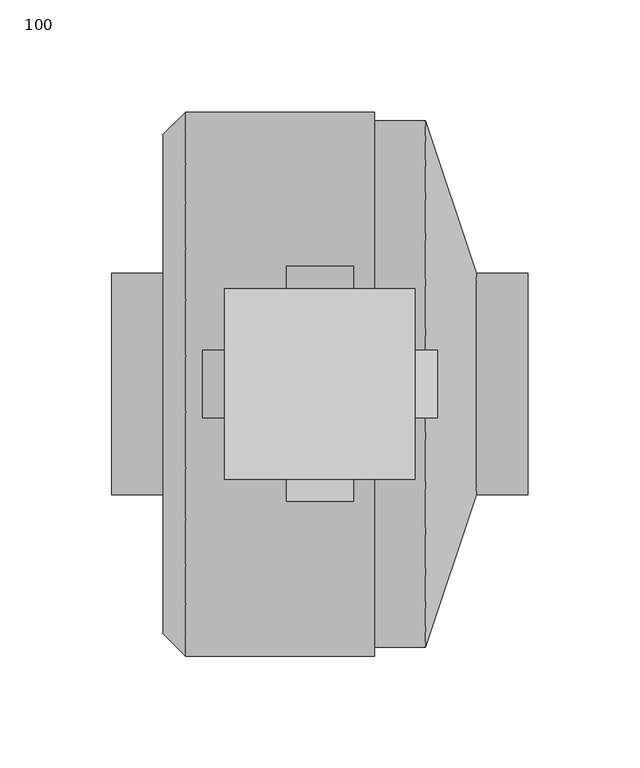
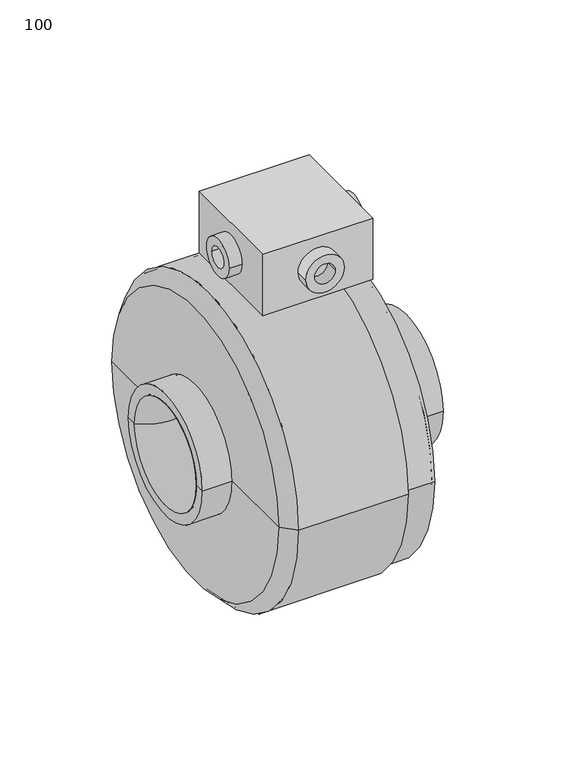
"""IFC4 building model written with IfcOpenShell, lengths in millimetres: proxy geometry, ВЕЗА_Канал-ВЕНТ : 100."""

from ifc_helpers import new_model, si_unit, point, frame, frame_2d, origin, place, context, project, spatial, polyline, circle_curve, ellipse_curve, trimmed, segment, composite_curve, outline, extrude, source, transform, mapped, element, save
from ifc_brep_helpers import plane_surface, cylinder_surface, revolved_surface, advanced_brep


def proxy_100_a4e0c5e0(model_context):
    return source(origin(), model_context, "Body", "SolidModel", [
        extrude(outline(composite_curve([segment(trimmed(circle_curve(frame_2d((0.0, 147.0)), 15.0), [point((-15.0, 147.0))], [point((15.0, 147.0))], False, "CARTESIAN"), True, "CONTINUOUS"), segment(trimmed(circle_curve(frame_2d((0.0, 147.0)), 15.0), [point((15.0, 147.0))], [point((-15.0, 147.0))], False, "CARTESIAN"), True, "CONTINUOUS")], self_intersect=False), holes=[composite_curve([segment(trimmed(circle_curve(frame_2d((0.0, 147.0)), 8.0), [point((-8.0, 147.0))], [point((8.0, 147.0))], True, "CARTESIAN"), True, "CONTINUOUS"), segment(trimmed(circle_curve(frame_2d((0.0, 147.0)), 8.0), [point((8.0, 147.0))], [point((-8.0, 147.0))], True, "CARTESIAN"), True, "CONTINUOUS")], self_intersect=False)]), frame((42.5, 0.0, 0.0), z_axis=(1.0, 0.0, 0.0), x_axis=(0.0, 1.0, 0.0)), (0.0, 0.0, 1.0), 10.0),
        extrude(outline(composite_curve([segment(trimmed(circle_curve(frame_2d((0.0, 147.0)), 15.0), [point((-15.0, 147.0))], [point((15.0, 147.0))], False, "CARTESIAN"), True, "CONTINUOUS"), segment(trimmed(circle_curve(frame_2d((0.0, 147.0)), 15.0), [point((15.0, 147.0))], [point((-15.0, 147.0))], False, "CARTESIAN"), True, "CONTINUOUS")], self_intersect=False), holes=[composite_curve([segment(trimmed(circle_curve(frame_2d((0.0, 147.0)), 8.0), [point((-8.0, 147.0))], [point((8.0, 147.0))], True, "CARTESIAN"), True, "CONTINUOUS"), segment(trimmed(circle_curve(frame_2d((0.0, 147.0)), 8.0), [point((8.0, 147.0))], [point((-8.0, 147.0))], True, "CARTESIAN"), True, "CONTINUOUS")], self_intersect=False)]), frame((-52.5, 0.0, 0.0), z_axis=(1.0, 0.0, 0.0), x_axis=(0.0, 1.0, 0.0)), (0.0, 0.0, 1.0), 10.0),
        extrude(outline(composite_curve([segment(trimmed(circle_curve(frame_2d((147.0, 0.0)), 15.0), [point((147.0, 15.0))], [point((147.0, -15.0))], False, "CARTESIAN"), True, "CONTINUOUS"), segment(trimmed(circle_curve(frame_2d((147.0, 0.0)), 15.0), [point((147.0, -15.0))], [point((147.0, 15.0))], False, "CARTESIAN"), True, "CONTINUOUS")], self_intersect=False), holes=[composite_curve([segment(trimmed(circle_curve(frame_2d((147.0, 0.0)), 8.0), [point((147.0, 8.0))], [point((147.0, -8.0))], True, "CARTESIAN"), True, "CONTINUOUS"), segment(trimmed(circle_curve(frame_2d((147.0, 0.0)), 8.0), [point((147.0, -8.0))], [point((147.0, 8.0))], True, "CARTESIAN"), True, "CONTINUOUS")], self_intersect=False)]), frame((0.0, -52.5, 0.0), z_axis=(0.0, 1.0, 0.0), x_axis=(0.0, 0.0, 1.0)), (0.0, 0.0, 1.0), 10.0),
        extrude(outline(composite_curve([segment(trimmed(circle_curve(frame_2d((147.0, 0.0)), 15.0), [point((147.0, 15.0))], [point((147.0, -15.0))], False, "CARTESIAN"), True, "CONTINUOUS"), segment(trimmed(circle_curve(frame_2d((147.0, 0.0)), 15.0), [point((147.0, -15.0))], [point((147.0, 15.0))], False, "CARTESIAN"), True, "CONTINUOUS")], self_intersect=False), holes=[composite_curve([segment(trimmed(circle_curve(frame_2d((147.0, 0.0)), 8.0), [point((147.0, 8.0))], [point((147.0, -8.0))], True, "CARTESIAN"), True, "CONTINUOUS"), segment(trimmed(circle_curve(frame_2d((147.0, 0.0)), 8.0), [point((147.0, -8.0))], [point((147.0, 8.0))], True, "CARTESIAN"), True, "CONTINUOUS")], self_intersect=False)]), frame((0.0, 42.5, 0.0), z_axis=(0.0, 1.0, 0.0), x_axis=(0.0, 0.0, 1.0)), (0.0, 0.0, 1.0), 10.0),
        extrude(outline(polyline([(-42.5, -42.5), (-42.5, 42.5), (42.5, 42.5), (42.5, -42.5), (-42.5, -42.5)])), frame((0.0, 0.0, 121.5), z_axis=(0.0, 0.0, 1.0), x_axis=(1.0, 0.0, 0.0)), (0.0, 0.0, 1.0), 50.0),
        advanced_brep(
        [(-93.0, -41.5, 0.0), (-93.0, 41.5, 0.0), (-91.5, 41.5, 0.0), (-91.5, -41.5, 0.0), (-48.0, -41.5, 0.0), (-48.0, 41.5, 0.0), (-49.5, -41.5, 0.0), (-49.5, 41.5, 0.0)],
        [
            (0, 1, circle_curve(frame((-93.0, 0.0, 0.0), z_axis=(1.0, 0.0, 0.0), x_axis=(0.0, 1.0, 0.0)), 41.5)),
            (1, 2),
            (2, 3, circle_curve(frame((-91.5, 0.0, 0.0), z_axis=(-1.0, 0.0, 0.0), x_axis=(0.0, 1.0, 0.0)), 41.5)),
            (3, 0),
            (1, 0, circle_curve(frame((-93.0, 0.0, 0.0), z_axis=(1.0, 0.0, 0.0), x_axis=(0.0, 1.0, 0.0)), 41.5)),
            (3, 2, circle_curve(frame((-91.5, 0.0, 0.0), z_axis=(-1.0, 0.0, 0.0), x_axis=(0.0, 1.0, 0.0)), 41.5)),
            (4, 5, circle_curve(frame((-48.0, 0.0, 0.0), z_axis=(1.0, 0.0, 0.0), x_axis=(0.0, 1.0, 0.0)), 41.5)),
            (5, 1, circle_curve(frame((-70.5, 65.1335583, 0.0), z_axis=(0.0, 0.0, -1.0), x_axis=(1.0, 0.0, 0.0)), 32.6311979)),
            (0, 4, circle_curve(frame((-70.5, -65.1335583, 0.0), z_axis=(0.0, 0.0, -1.0), x_axis=(1.0, 0.0, 0.0)), 32.6311979)),
            (5, 4, circle_curve(frame((-48.0, 0.0, 0.0), z_axis=(1.0, 0.0, 0.0), x_axis=(0.0, 1.0, 0.0)), 41.5)),
            (6, 7, circle_curve(frame((-49.5, 0.0, 0.0), z_axis=(1.0, 0.0, 0.0), x_axis=(0.0, 1.0, 0.0)), 41.5)),
            (7, 5),
            (4, 6),
            (7, 6, circle_curve(frame((-49.5, 0.0, 0.0), z_axis=(1.0, 0.0, 0.0), x_axis=(0.0, 1.0, 0.0)), 41.5)),
            (2, 7, circle_curve(frame((-70.5, 65.2023679, 0.0), z_axis=(0.0, 0.0, 1.0), x_axis=(1.0, 0.0, 0.0)), 31.667053)),
            (6, 3, circle_curve(frame((-70.5, -65.2023679, 0.0), z_axis=(0.0, 0.0, 1.0), x_axis=(1.0, 0.0, 0.0)), 31.667053)),
        ],
        [
            cylinder_surface(frame((-138.0, 0.0, 0.0), z_axis=(-1.0, 0.0, 0.0), x_axis=(0.0, 1.0, 0.0)), 41.5),
            revolved_surface(trimmed(ellipse_curve(frame((-70.5, 65.1335583, 0.0), z_axis=(0.0, 0.0, 1.0), x_axis=(1.0, 0.0, 0.0)), 32.6311979, 32.6311979), [point((-93.0, 41.5, 0.0))], [point((-48.0, 41.5, 0.0))], True, "CARTESIAN"), (-138.0, 0.0, 0.0), (-1.0, 0.0, 0.0)),
            revolved_surface(trimmed(ellipse_curve(frame((-70.5, 65.2023679, 0.0), z_axis=(0.0, 0.0, -1.0), x_axis=(1.0, 0.0, 0.0)), 31.667053, 31.667053), [point((-49.5, 41.5, 0.0))], [point((-91.5, 41.5, 0.0))], True, "CARTESIAN"), (-138.0, 0.0, 0.0), (-1.0, 0.0, 0.0)),
        ],
        [
            (0, [[1, 2, 3, 4]]),
            (0, [[5, -4, 6, -2]]),
            (1, [[7, 8, -1, 9]]),
            (1, [[10, -9, -5, -8]]),
            (0, [[11, 12, -7, 13]]),
            (0, [[14, -13, -10, -12]]),
            (2, [[-3, 15, -11, 16]]),
            (2, [[-6, -16, -14, -15]]),
        ],
    ),
        advanced_brep(
        [(-91.5, -48.0, 0.0), (-91.5, 48.0, 0.0), (-91.5, 41.5, 0.0), (-91.5, -41.5, 0.0), (22.8333333, -120.0, 0.0), (22.8333333, 120.0, 0.0), (-60.0, 120.0, 0.0), (-60.0, -120.0, 0.0), (22.8333333, -116.0, 0.0), (22.8333333, 116.0, 0.0), (45.6666667, -116.0, 0.0), (45.6666667, 116.0, 0.0), (68.5, -48.0, 0.0), (68.5, 48.0, 0.0), (93.0, -48.0, 0.0), (93.0, 48.0, 0.0), (93.0, -49.5, 0.0), (93.0, 49.5, 0.0), (70.0, -49.5, 0.0), (70.0, 49.5, 0.0), (47.1666667, -117.5, 0.0), (47.1666667, 117.5, 0.0), (24.3333333, -117.5, 0.0), (24.3333333, 117.5, 0.0), (24.3333333, -121.5, 0.0), (24.3333333, 121.5, 0.0), (-60.0, -121.5, 0.0), (-60.0, 121.5, 0.0), (-70.0, -49.5, 0.0), (-70.0, 49.5, 0.0), (-70.0, 111.5, 0.0), (-70.0, -111.5, 0.0), (-93.0, -49.5, 0.0), (-93.0, 49.5, 0.0), (-93.0, -41.5, 0.0), (-93.0, 41.5, 0.0), (-68.5, -48.0, 0.0), (-68.5, 48.0, 0.0), (-68.5, -111.5, 0.0), (-68.5, 111.5, 0.0)],
        [
            (0, 1, circle_curve(frame((-91.5, 0.0, 0.0), z_axis=(1.0, 0.0, 0.0), x_axis=(0.0, 1.0, 0.0)), 48.0)),
            (1, 2),
            (2, 3, circle_curve(frame((-91.5, 0.0, 0.0), z_axis=(-1.0, 0.0, 0.0), x_axis=(0.0, 1.0, 0.0)), 41.5)),
            (3, 0),
            (1, 0, circle_curve(frame((-91.5, 0.0, 0.0), z_axis=(1.0, 0.0, 0.0), x_axis=(0.0, 1.0, 0.0)), 48.0)),
            (3, 2, circle_curve(frame((-91.5, 0.0, 0.0), z_axis=(-1.0, 0.0, 0.0), x_axis=(0.0, 1.0, 0.0)), 41.5)),
            (4, 5, circle_curve(frame((22.8333333, 0.0, 0.0), z_axis=(1.0, 0.0, 0.0), x_axis=(0.0, 1.0, 0.0)), 120.0)),
            (5, 6),
            (6, 7, circle_curve(frame((-60.0, 0.0, 0.0), z_axis=(-1.0, 0.0, 0.0), x_axis=(0.0, 1.0, 0.0)), 120.0)),
            (7, 4),
            (5, 4, circle_curve(frame((22.8333333, 0.0, 0.0), z_axis=(1.0, 0.0, 0.0), x_axis=(0.0, 1.0, 0.0)), 120.0)),
            (7, 6, circle_curve(frame((-60.0, 0.0, 0.0), z_axis=(-1.0, 0.0, 0.0), x_axis=(0.0, 1.0, 0.0)), 120.0)),
            (8, 9, circle_curve(frame((22.8333333, 0.0, 0.0), z_axis=(1.0, 0.0, 0.0), x_axis=(0.0, 1.0, 0.0)), 116.0)),
            (9, 5),
            (4, 8),
            (9, 8, circle_curve(frame((22.8333333, 0.0, 0.0), z_axis=(1.0, 0.0, 0.0), x_axis=(0.0, 1.0, 0.0)), 116.0)),
            (10, 11, circle_curve(frame((45.6666667, 0.0, 0.0), z_axis=(1.0, 0.0, 0.0), x_axis=(0.0, 1.0, 0.0)), 116.0)),
            (11, 9),
            (8, 10),
            (11, 10, circle_curve(frame((45.6666667, 0.0, 0.0), z_axis=(1.0, 0.0, 0.0), x_axis=(0.0, 1.0, 0.0)), 116.0)),
            (12, 13, circle_curve(frame((68.5, 0.0, 0.0), z_axis=(1.0, 0.0, 0.0), x_axis=(0.0, 1.0, 0.0)), 48.0)),
            (13, 11),
            (10, 12),
            (13, 12, circle_curve(frame((68.5, 0.0, 0.0), z_axis=(1.0, 0.0, 0.0), x_axis=(0.0, 1.0, 0.0)), 48.0)),
            (14, 15, circle_curve(frame((93.0, 0.0, 0.0), z_axis=(1.0, 0.0, 0.0), x_axis=(0.0, 1.0, 0.0)), 48.0)),
            (15, 13),
            (12, 14),
            (15, 14, circle_curve(frame((93.0, 0.0, 0.0), z_axis=(1.0, 0.0, 0.0), x_axis=(0.0, 1.0, 0.0)), 48.0)),
            (16, 17, circle_curve(frame((93.0, 0.0, 0.0), z_axis=(1.0, 0.0, 0.0), x_axis=(0.0, 1.0, 0.0)), 49.5)),
            (17, 15),
            (14, 16),
            (17, 16, circle_curve(frame((93.0, 0.0, 0.0), z_axis=(1.0, 0.0, 0.0), x_axis=(0.0, 1.0, 0.0)), 49.5)),
            (18, 19, circle_curve(frame((70.0, 0.0, 0.0), z_axis=(1.0, 0.0, 0.0), x_axis=(0.0, 1.0, 0.0)), 49.5)),
            (19, 17),
            (16, 18),
            (19, 18, circle_curve(frame((70.0, 0.0, 0.0), z_axis=(1.0, 0.0, 0.0), x_axis=(0.0, 1.0, 0.0)), 49.5)),
            (20, 21, circle_curve(frame((47.1666667, 0.0, 0.0), z_axis=(1.0, 0.0, 0.0), x_axis=(0.0, 1.0, 0.0)), 117.5)),
            (21, 19),
            (18, 20),
            (21, 20, circle_curve(frame((47.1666667, 0.0, 0.0), z_axis=(1.0, 0.0, 0.0), x_axis=(0.0, 1.0, 0.0)), 117.5)),
            (22, 23, circle_curve(frame((24.3333333, 0.0, 0.0), z_axis=(1.0, 0.0, 0.0), x_axis=(0.0, 1.0, 0.0)), 117.5)),
            (23, 21),
            (20, 22),
            (23, 22, circle_curve(frame((24.3333333, 0.0, 0.0), z_axis=(1.0, 0.0, 0.0), x_axis=(0.0, 1.0, 0.0)), 117.5)),
            (24, 25, circle_curve(frame((24.3333333, 0.0, 0.0), z_axis=(1.0, 0.0, 0.0), x_axis=(0.0, 1.0, 0.0)), 121.5)),
            (25, 23),
            (22, 24),
            (25, 24, circle_curve(frame((24.3333333, 0.0, 0.0), z_axis=(1.0, 0.0, 0.0), x_axis=(0.0, 1.0, 0.0)), 121.5)),
            (26, 27, circle_curve(frame((-60.0, 0.0, 0.0), z_axis=(1.0, 0.0, 0.0), x_axis=(0.0, 1.0, 0.0)), 121.5)),
            (27, 25),
            (24, 26),
            (27, 26, circle_curve(frame((-60.0, 0.0, 0.0), z_axis=(1.0, 0.0, 0.0), x_axis=(0.0, 1.0, 0.0)), 121.5)),
            (28, 29, circle_curve(frame((-70.0, 0.0, 0.0), z_axis=(1.0, 0.0, 0.0), x_axis=(0.0, 1.0, 0.0)), 49.5)),
            (29, 30),
            (30, 31, circle_curve(frame((-70.0, 0.0, 0.0), z_axis=(-1.0, 0.0, 0.0), x_axis=(0.0, 1.0, 0.0)), 111.5)),
            (31, 28),
            (29, 28, circle_curve(frame((-70.0, 0.0, 0.0), z_axis=(1.0, 0.0, 0.0), x_axis=(0.0, 1.0, 0.0)), 49.5)),
            (31, 30, circle_curve(frame((-70.0, 0.0, 0.0), z_axis=(-1.0, 0.0, 0.0), x_axis=(0.0, 1.0, 0.0)), 111.5)),
            (32, 33, circle_curve(frame((-93.0, 0.0, 0.0), z_axis=(1.0, 0.0, 0.0), x_axis=(0.0, 1.0, 0.0)), 49.5)),
            (33, 29),
            (28, 32),
            (33, 32, circle_curve(frame((-93.0, 0.0, 0.0), z_axis=(1.0, 0.0, 0.0), x_axis=(0.0, 1.0, 0.0)), 49.5)),
            (34, 35, circle_curve(frame((-93.0, 0.0, 0.0), z_axis=(1.0, 0.0, 0.0), x_axis=(0.0, 1.0, 0.0)), 41.5)),
            (35, 33),
            (32, 34),
            (35, 34, circle_curve(frame((-93.0, 0.0, 0.0), z_axis=(1.0, 0.0, 0.0), x_axis=(0.0, 1.0, 0.0)), 41.5)),
            (2, 35),
            (34, 3),
            (36, 37, circle_curve(frame((-68.5, 0.0, 0.0), z_axis=(1.0, 0.0, 0.0), x_axis=(0.0, 1.0, 0.0)), 48.0)),
            (37, 1),
            (0, 36),
            (37, 36, circle_curve(frame((-68.5, 0.0, 0.0), z_axis=(1.0, 0.0, 0.0), x_axis=(0.0, 1.0, 0.0)), 48.0)),
            (38, 39, circle_curve(frame((-68.5, 0.0, 0.0), z_axis=(1.0, 0.0, 0.0), x_axis=(0.0, 1.0, 0.0)), 111.5)),
            (39, 37),
            (36, 38),
            (39, 38, circle_curve(frame((-68.5, 0.0, 0.0), z_axis=(1.0, 0.0, 0.0), x_axis=(0.0, 1.0, 0.0)), 111.5)),
            (6, 39),
            (38, 7),
            (30, 27),
            (26, 31),
        ],
        [
            plane_surface(frame((-91.5, 0.0, 0.0), z_axis=(1.0, 0.0, 0.0), x_axis=(0.0, 1.0, 0.0))),
            revolved_surface(polyline([(-60.0, 120.0, 0.0), (22.833333299999993, 120.0, 0.0)]), (-163.0, 0.0, 0.0), (-1.0, 0.0, 0.0)),
            plane_surface(frame((22.8333333, 0.0, 0.0), z_axis=(-1.0, 0.0, 0.0), x_axis=(0.0, 1.0, 0.0))),
            revolved_surface(polyline([(22.833333299999993, 116.0, 0.0), (45.66666670000001, 116.0, 0.0)]), (-163.0, 0.0, 0.0), (-1.0, 0.0, 0.0)),
            revolved_surface(polyline([(45.6666667, 116.0, 0.0), (68.5, 48.0, 0.0)]), (-163.0, 0.0, 0.0), (-1.0, 0.0, 0.0)),
            revolved_surface(polyline([(68.5, 48.0, 0.0), (93.0, 48.0, 0.0)]), (-163.0, 0.0, 0.0), (-1.0, 0.0, 0.0)),
            plane_surface(frame((93.0, 0.0, 0.0), z_axis=(1.0, 0.0, 0.0), x_axis=(0.0, 1.0, 0.0))),
            cylinder_surface(frame((-163.0, 0.0, 0.0), z_axis=(-1.0, 0.0, 0.0), x_axis=(0.0, 1.0, 0.0)), 49.5),
            revolved_surface(polyline([(70.0, 49.5, 0.0), (47.1666667, 117.5, 0.0)]), (-163.0, 0.0, 0.0), (-1.0, 0.0, 0.0)),
            cylinder_surface(frame((-163.0, 0.0, 0.0), z_axis=(-1.0, 0.0, 0.0), x_axis=(0.0, 1.0, 0.0)), 117.5),
            plane_surface(frame((24.3333333, 0.0, 0.0), z_axis=(1.0, 0.0, 0.0), x_axis=(0.0, 1.0, 0.0))),
            cylinder_surface(frame((-163.0, 0.0, 0.0), z_axis=(-1.0, 0.0, 0.0), x_axis=(0.0, 1.0, 0.0)), 121.5),
            plane_surface(frame((-70.0, 0.0, 0.0), z_axis=(-1.0, 0.0, 0.0), x_axis=(0.0, 1.0, 0.0))),
            plane_surface(frame((-93.0, 0.0, 0.0), z_axis=(-1.0, 0.0, 0.0), x_axis=(0.0, 1.0, 0.0))),
            revolved_surface(polyline([(-93.0, 41.5, 0.0), (-91.5, 41.5, 0.0)]), (-163.0, 0.0, 0.0), (-1.0, 0.0, 0.0)),
            revolved_surface(polyline([(-91.5, 48.0, 0.0), (-68.5, 48.0, 0.0)]), (-163.0, 0.0, 0.0), (-1.0, 0.0, 0.0)),
            plane_surface(frame((-68.5, 0.0, 0.0), z_axis=(1.0, 0.0, 0.0), x_axis=(0.0, 1.0, 0.0))),
            revolved_surface(polyline([(-68.5, 111.5, 0.0), (-60.0, 120.0, 0.0)]), (-163.0, 0.0, 0.0), (-1.0, 0.0, 0.0)),
            revolved_surface(polyline([(-60.0, 121.5, 0.0), (-70.0, 111.5, 0.0)]), (-163.0, 0.0, 0.0), (-1.0, 0.0, 0.0)),
        ],
        [
            (0, [[1, 2, 3, 4]]),
            (0, [[5, -4, 6, -2]]),
            (1, [[7, 8, 9, 10]]),
            (1, [[11, -10, 12, -8]]),
            (2, [[13, 14, -7, 15]]),
            (2, [[16, -15, -11, -14]]),
            (3, [[17, 18, -13, 19]]),
            (3, [[20, -19, -16, -18]]),
            (4, [[21, 22, -17, 23]]),
            (4, [[24, -23, -20, -22]]),
            (5, [[25, 26, -21, 27]]),
            (5, [[28, -27, -24, -26]]),
            (6, [[29, 30, -25, 31]]),
            (6, [[32, -31, -28, -30]]),
            (7, [[33, 34, -29, 35]]),
            (7, [[36, -35, -32, -34]]),
            (8, [[37, 38, -33, 39]]),
            (8, [[40, -39, -36, -38]]),
            (9, [[41, 42, -37, 43]]),
            (9, [[44, -43, -40, -42]]),
            (10, [[45, 46, -41, 47]]),
            (10, [[48, -47, -44, -46]]),
            (11, [[49, 50, -45, 51]]),
            (11, [[52, -51, -48, -50]]),
            (12, [[53, 54, 55, 56]]),
            (12, [[57, -56, 58, -54]]),
            (7, [[59, 60, -53, 61]]),
            (7, [[62, -61, -57, -60]]),
            (13, [[63, 64, -59, 65]]),
            (13, [[66, -65, -62, -64]]),
            (14, [[-3, 67, -63, 68]]),
            (14, [[-6, -68, -66, -67]]),
            (15, [[69, 70, -1, 71]]),
            (15, [[72, -71, -5, -70]]),
            (16, [[73, 74, -69, 75]]),
            (16, [[76, -75, -72, -74]]),
            (17, [[-9, 77, -73, 78]]),
            (17, [[-12, -78, -76, -77]]),
            (18, [[-55, 79, -49, 80]]),
            (18, [[-58, -80, -52, -79]]),
        ],
    ),
        advanced_brep(
        [(0.0, -85.5, 0.0), (0.0, 85.5, 0.0), (0.0, 0.0, 0.0), (-48.0, -85.5, 0.0), (-48.0, 85.5, 0.0), (-48.0, 0.0, 0.0)],
        [
            (0, 1, circle_curve(frame((0.0, 0.0, 0.0), z_axis=(1.0, 0.0, 0.0), x_axis=(0.0, 1.0, 0.0)), 85.5)),
            (1, 2),
            (2, 0),
            (1, 0, circle_curve(frame((0.0, 0.0, 0.0), z_axis=(1.0, 0.0, 0.0), x_axis=(0.0, 1.0, 0.0)), 85.5)),
            (3, 4, circle_curve(frame((-48.0, 0.0, 0.0), z_axis=(1.0, 0.0, 0.0), x_axis=(0.0, 1.0, 0.0)), 85.5)),
            (4, 1),
            (0, 3),
            (4, 3, circle_curve(frame((-48.0, 0.0, 0.0), z_axis=(1.0, 0.0, 0.0), x_axis=(0.0, 1.0, 0.0)), 85.5)),
            (5, 4),
            (3, 5),
        ],
        [
            plane_surface(frame((0.0, 0.0, 0.0), z_axis=(1.0, 0.0, 0.0), x_axis=(0.0, 1.0, 0.0))),
            cylinder_surface(frame((-183.0, 0.0, 0.0), z_axis=(-1.0, 0.0, 0.0), x_axis=(0.0, 1.0, 0.0)), 85.5),
            plane_surface(frame((-48.0, 0.0, 0.0), z_axis=(-1.0, 0.0, 0.0), x_axis=(0.0, 1.0, 0.0))),
        ],
        [
            (0, [[1, 2, 3]]),
            (0, [[4, -3, -2]]),
            (1, [[5, 6, -1, 7]]),
            (1, [[8, -7, -4, -6]]),
            (2, [[9, -5, 10]]),
            (2, [[-10, -8, -9]]),
        ],
    ),
    ])


if __name__ == "__main__":
    model = new_model("IFC4")
    model_context = context("Model", 3, world=origin())
    ifc_project = project(units=[si_unit("LENGTHUNIT", "METRE", prefix="MILLI")], contexts=[model_context])
    site = spatial("IfcSite", under=ifc_project)
    building = spatial("IfcBuilding", under=site)
    placement = place(None, origin())
    proxy_100_shape = proxy_100_a4e0c5e0(model_context)
    element("IfcBuildingElementProxy", 1, Name="ВЕЗА_Канал-ВЕНТ : 100", ObjectType="ВЕЗА_Канал-ВЕНТ : 100", at=placement, inside=building, context=model_context, shape_type="MappedRepresentation", body=[
        mapped(proxy_100_shape, transform((0.0, 0.0, 0.0), x_axis=(1.0, 0.0, 0.0), y_axis=(0.0, 1.0, 0.0), z_axis=(0.0, 0.0, 1.0))),
    ])
    save(model, "model.ifc")

# Revit data of these elements
# Type "ВЕЗА_Канал-ВЕНТ : 100"
#   ВЕЗА_Классификатор = "11031"
#   ВЕЗА_Контакты = "bim@veza.ru"
#   URL = "http://www.veza.ru/docs/sistemy-kanalnoy-ventilyatsii-kanal/"
#   Таблица = "kanal-vent"
#   ADSK_Примечание = ""
#   ADSK_Позиция на схеме = ""
#   ADSK_Позиция = "3"
#   ADSK_Наименование краткое = "Канал-ВЕНТ"
#   ADSK_Наименование = "Вентилятор канальный для круглых каналов, потребляемая мощность электродвигателя N=0,065 кВт, частота вращения двигателя n=2400об/мин, напряжение сети 230В"
#   ADSK_Марка = "Канал-ВЕНТ-100 ТУ 4861-155-40149153-2010"
#   ADSK_Комплект [instance default] = ""
#   ADSK_Код изделия = ""
#   ADSK_Завод-изготовитель = "ООО \"Веза\", Россия, Москва, ИНН 505001001, info@veza.ru"
#   ADSK_Единица измерения = "компл."
#   ADSK_Дата изменения = "10.03.2020"
#   ADSK_Группирование = ""
#   ADSK_Версия семейства = "Версия 4"
#   ADSK_Версия Revit = "Revit 2017"
#   Угол поворота УГО 3D [instance default] = 45°
#   L [instance default] = 186 mm
#   h [instance default] = 23 mm
#   D [instance default] = 243 mm
#   ADSK_Ток [instance default] = 0.29 A
#   ADSK_Расход воздуха [instance default] = 561.6 m³/h
#   ADSK_Размер_Диаметр [instance default] = 99 mm
#   ADSK_Полная мощность [instance default] = 65 VA
#   ADSK_Номинальная мощность [instance default] = 65 W
#   ADSK_Напряжение = 230 V
#   ADSK_Масса [instance default] = 3.2
#   ADSK_Коэффициент мощности = 1
#   ADSK_Количество = 1
#   Масштаб УГО [instance default] = 100
#   ВЕЗА_Типоразмер = 100
#   ВЕЗА_Число полюсов = 2
#   ADSK_Частота вращения двигателя [instance default] = 2400
#   ADSK_Количество фаз = 1
#   Материал = ВЕЗА_Оцинкованная сталь
#   Default Elevation = 0
#   Description = (empty or 0)
#   Type Image = (empty or 0)
#   Manufacturer = ""
# Element 1 (IfcBuildingElementProxy, "ВЕЗА_Канал-ВЕНТ : 100")
#   Materials on its faces: "ВЕЗА_Оцинкованная сталь", "Пластмасса коробки"
# Materials
#   "ВЕЗА_Оцинкованная сталь": class "Типовые", colour RGB 120 120 120, transparency 0, Cost = 0
#   "Пластмасса коробки": class "Типовые", colour RGB 120 120 120, transparency 0, Cost = 0
